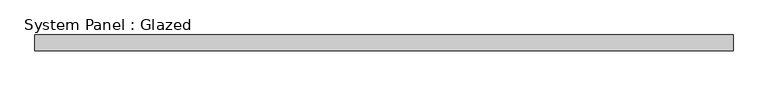
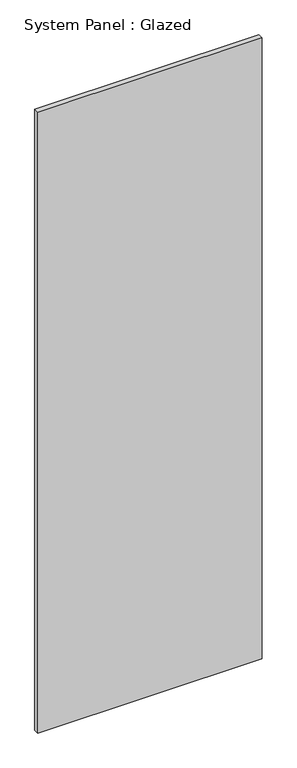
"""IFC4 building model written with IfcOpenShell, lengths in millimetres: plate geometry, System Panel : Glazed."""

import ifcopenshell
import ifcopenshell.guid

model = None  # the IFC model being written
_history = None  # IfcOwnerHistory: only IFC2X3 demands one
_inside = {}  # id of a spatial element -> (the spatial element, [elements in it])
_under = {}  # id of a project, library or spatial element -> (it, [spatial elements below it])
_declared = {}  # id of a project -> (the project, [libraries it declares])
_typed = {}  # id of a type object -> (the type object, [elements of that type])
_made_of = {}  # id of a material, layer set ... -> (it, [elements and type objects made of it])


def new_model(schema):
    """Start an empty IFC model of exactly this schema.

    Asked for "IFC4X3", IfcOpenShell would pick the latest addendum, in which some entities
    have other attributes; the version numbers below select the first issue.
    IFC2X3 requires an IfcOwnerHistory on every rooted entity: one is made here for all.
    """
    global model, _history
    if schema == "IFC4X3":
        model = ifcopenshell.file(schema_version=(4, 3, 0, 0))
    else:
        model = ifcopenshell.file(schema=schema)
    _inside.clear()
    _under.clear()
    _declared.clear()
    _typed.clear()
    _made_of.clear()
    _history = None
    if model.schema == "IFC2X3":
        org = make("IfcOrganization", Name="unknown")
        user = make(
            "IfcPersonAndOrganization",
            ThePerson=make("IfcPerson", FamilyName="unknown"),
            TheOrganization=org,
        )
        app = make(
            "IfcApplication",
            ApplicationDeveloper=org,
            Version="unknown",
            ApplicationFullName="unknown",
            ApplicationIdentifier="unknown",
        )
        _history = make(
            "IfcOwnerHistory",
            OwningUser=user,
            OwningApplication=app,
            ChangeAction="ADDED",
            CreationDate=0,
        )
    return model


def make(cls, **values):
    """One entity of the class cls with the attributes given. An attribute that is None is left unset."""
    return model.create_entity(
        cls, **{name: value for name, value in values.items() if value is not None}
    )


def rooted(cls, **values):
    """An entity with a GlobalId (a new one), such as an element, a storey or a relation."""
    return make(cls, GlobalId=ifcopenshell.guid.new(), OwnerHistory=_history, **values)


def si_unit(unit_type, name, prefix=None):
    """IfcSIUnit, for example si_unit("LENGTHUNIT", "METRE", prefix="MILLI")."""
    return make("IfcSIUnit", UnitType=unit_type, Prefix=prefix, Name=name)


def assignment(units):
    """IfcUnitAssignment: the units of a project."""
    return None if units is None else make("IfcUnitAssignment", Units=units)


def point(xyz):
    """IfcCartesianPoint."""
    return None if xyz is None else make("IfcCartesianPoint", Coordinates=xyz)


def direction(xyz):
    """IfcDirection."""
    return None if xyz is None else make("IfcDirection", DirectionRatios=xyz)


def frame(location, z_axis=None, x_axis=None):
    """IfcAxis2Placement3D, a coordinate frame: its origin and axes. An axis left out is left unset."""
    return make(
        "IfcAxis2Placement3D",
        Location=point(location),
        Axis=direction(z_axis),
        RefDirection=direction(x_axis),
    )


def origin():
    """The frame at (0, 0, 0) with its axes left unset."""
    return frame((0.0, 0.0, 0.0))


def origin_with_axes():
    """The frame at (0, 0, 0) with the z axis (0, 0, 1) and the x axis (1, 0, 0) written out."""
    return frame((0.0, 0.0, 0.0), z_axis=(0.0, 0.0, 1.0), x_axis=(1.0, 0.0, 0.0))


def place(relative_to, where):
    """IfcLocalPlacement: puts the frame where relative to a parent placement (None: the world)."""
    return make(
        "IfcLocalPlacement", PlacementRelTo=relative_to, RelativePlacement=where
    )


def context(
    kind, dimensions, precision=None, world=None, true_north=None, identifier=None
):
    """IfcGeometricRepresentationContext, for example the 3D "Model" context."""
    return make(
        "IfcGeometricRepresentationContext",
        ContextIdentifier=identifier,
        ContextType=kind,
        CoordinateSpaceDimension=dimensions,
        Precision=precision,
        WorldCoordinateSystem=world,
        TrueNorth=true_north,
    )


def project(units=None, contexts=None):
    """IfcProject with its units and contexts."""
    return rooted(
        "IfcProject",
        Name="project",
        RepresentationContexts=contexts,
        UnitsInContext=assignment(units),
    )


def spatial(cls, under=None, at=None, **own):
    """A site, building, storey or space (cls), placed at a placement, below another one or the project."""
    s = rooted(cls, ObjectPlacement=at, **own)
    if under is not None:
        _under.setdefault(under.id(), (under, []))[1].append(s)
    return s


def polyline(points):
    """IfcPolyline through the points."""
    return make("IfcPolyline", Points=[point(p) for p in points])


def outline(outer, holes=None, kind="AREA"):
    """IfcArbitraryClosedProfileDef: a profile drawn as a closed curve; with holes, ...WithVoids."""
    if holes is None:
        return make("IfcArbitraryClosedProfileDef", ProfileType=kind, OuterCurve=outer)
    return make(
        "IfcArbitraryProfileDefWithVoids",
        ProfileType=kind,
        OuterCurve=outer,
        InnerCurves=holes,
    )


def extrude(swept, where, along, depth):
    """IfcExtrudedAreaSolid: the profile swept, set in the frame where, extruded along a direction by depth."""
    return make(
        "IfcExtrudedAreaSolid",
        SweptArea=swept,
        Position=where,
        ExtrudedDirection=direction(along),
        Depth=depth,
    )


def shape(context_of_items, identifier, shape_type, items):
    """IfcShapeRepresentation: the items that make up one representation, for example the "Body"."""
    return make(
        "IfcShapeRepresentation",
        ContextOfItems=context_of_items,
        RepresentationIdentifier=identifier,
        RepresentationType=shape_type,
        Items=items,
    )


def source(mapping_origin, context_of_items, identifier, shape_type, items):
    """IfcRepresentationMap: a shape defined once, which mapped items show again and again."""
    return make(
        "IfcRepresentationMap",
        MappingOrigin=mapping_origin,
        MappedRepresentation=shape(context_of_items, identifier, shape_type, items),
    )


def transform(
    local_origin,
    x_axis=None,
    y_axis=None,
    z_axis=None,
    scale=None,
    scale2=None,
    scale3=None,
    uniform=True,
):
    """IfcCartesianTransformationOperator3D, or its non-uniform kind. x_axis, y_axis, z_axis: its Axis1, 2, 3."""
    if uniform:
        return make(
            "IfcCartesianTransformationOperator3D",
            Axis1=direction(x_axis),
            Axis2=direction(y_axis),
            LocalOrigin=point(local_origin),
            Scale=scale,
            Axis3=direction(z_axis),
        )
    return make(
        "IfcCartesianTransformationOperator3DnonUniform",
        Axis1=direction(x_axis),
        Axis2=direction(y_axis),
        LocalOrigin=point(local_origin),
        Scale=scale,
        Axis3=direction(z_axis),
        Scale2=scale2,
        Scale3=scale3,
    )


def mapped(mapping_source, mapping_target):
    """IfcMappedItem: shows the shape of a source again, moved by a transform."""
    return make(
        "IfcMappedItem", MappingSource=mapping_source, MappingTarget=mapping_target
    )


def made_of(thing, what):
    """Note that an element or type object is made of a material, layer set ...; save() writes the relation."""
    if what is not None:
        _made_of.setdefault(what.id(), (what, []))[1].append(thing)
    return thing


def element(
    cls,
    number,
    at=None,
    inside=None,
    cuts=None,
    type_object=None,
    material=None,
    context=None,
    identifier="Body",
    shape_type=None,
    held_by="IfcProductDefinitionShape",
    body=None,
    shapes=None,
    **own,
):
    """One element of the class cls, such as IfcWall. Its Tag is "e" and its number.

    at: its placement. inside: the storey or other place that contains it. cuts: it is an
    opening in that element (IfcRelVoidsElement). A single representation is given by context,
    identifier, shape_type and body (its items); several are given by shapes. held_by: the class
    of the entity that holds the representations. save() writes the other relations.
    """
    e = rooted(cls, Tag="e%d" % number, ObjectPlacement=at, **own)
    if body is not None:
        shapes = [shape(context, identifier, shape_type, body)]
    if shapes is not None:
        e.Representation = make(held_by, Representations=shapes)
    if inside is not None:
        _inside.setdefault(inside.id(), (inside, []))[1].append(e)
    if cuts is not None:
        rooted(
            "IfcRelVoidsElement", RelatingBuildingElement=cuts, RelatedOpeningElement=e
        )
    if type_object is not None:
        _typed.setdefault(type_object.id(), (type_object, []))[1].append(e)
    return made_of(e, material)


def aggregate(whole, parts):
    """IfcRelAggregates: a whole, such as a stair, and the parts it consists of."""
    return rooted("IfcRelAggregates", RelatingObject=whole, RelatedObjects=parts)


def save(model, path):
    """Write the relations noted so far, then the file.

    IfcRelAggregates (storeys below a building ...), IfcRelContainedInSpatialStructure (elements
    in a storey), IfcRelDefinesByType, IfcRelAssociatesMaterial and IfcRelDeclares: one each for
    every whole, place, type object, material and project.
    """
    for whole, parts in _under.values():
        aggregate(whole, parts)
    for where, things in _inside.values():
        rooted(
            "IfcRelContainedInSpatialStructure",
            RelatedElements=things,
            RelatingStructure=where,
        )
    for kind, things in _typed.values():
        rooted("IfcRelDefinesByType", RelatedObjects=things, RelatingType=kind)
    for what, things in _made_of.values():
        rooted("IfcRelAssociatesMaterial", RelatedObjects=things, RelatingMaterial=what)
    for by, libraries in _declared.values():
        rooted("IfcRelDeclares", RelatingContext=by, RelatedDefinitions=libraries)
    model.write(path)


def system_panel_glazed_b92d501e(model_context):
    return source(origin(), model_context, "Body", "SweptSolid", [
        extrude(outline(polyline([(567.2666667, 19.05), (-567.2666667, 19.05), (-567.2666667, 44.45), (567.2666667, 44.45), (567.2666667, 19.05)])), origin_with_axes(), (0.0, 0.0, 1.0), 3318.9333333),
    ])


if __name__ == "__main__":
    model = new_model("IFC4")
    model_context = context("Model", 3, world=origin())
    ifc_project = project(units=[si_unit("LENGTHUNIT", "METRE", prefix="MILLI")], contexts=[model_context])
    site = spatial("IfcSite", under=ifc_project)
    building = spatial("IfcBuilding", under=site)
    placement = place(None, origin())
    system_panel_glazed_shape = system_panel_glazed_b92d501e(model_context)
    element("IfcPlate", 1, ObjectType="System Panel : Glazed", at=placement, inside=building, context=model_context, shape_type="MappedRepresentation", body=[
        mapped(system_panel_glazed_shape, transform((0.0, 0.0, 0.0), x_axis=(1.0, 0.0, 0.0), y_axis=(0.0, 1.0, 0.0), z_axis=(0.0, 0.0, 1.0))),
    ])
    save(model, "model.ifc")

# Revit data of these elements
# Type "System Panel : Glazed"
#   Construction Type Id = "GSP4R"
#   Analytic Construction = "1/8 in Pilkington single glazing"
#   Visual Light Transmittance = 0.9
#   Solar Heat Gain Coefficient = 0.86
#   Heat Transfer Coefficient (U) = 1.18115 BTU/(h·ft²·°F)
#   Define Thermal Properties by = 1
# Element 1 (IfcPlate, "System Panel : Glazed")
#   Materials on its faces: "Glass"
# Materials
#   "Glass": class "Glass", colour RGB 0 128 192, transparency 0.75, Description = "Soda Lime Glass", Cost = 0
